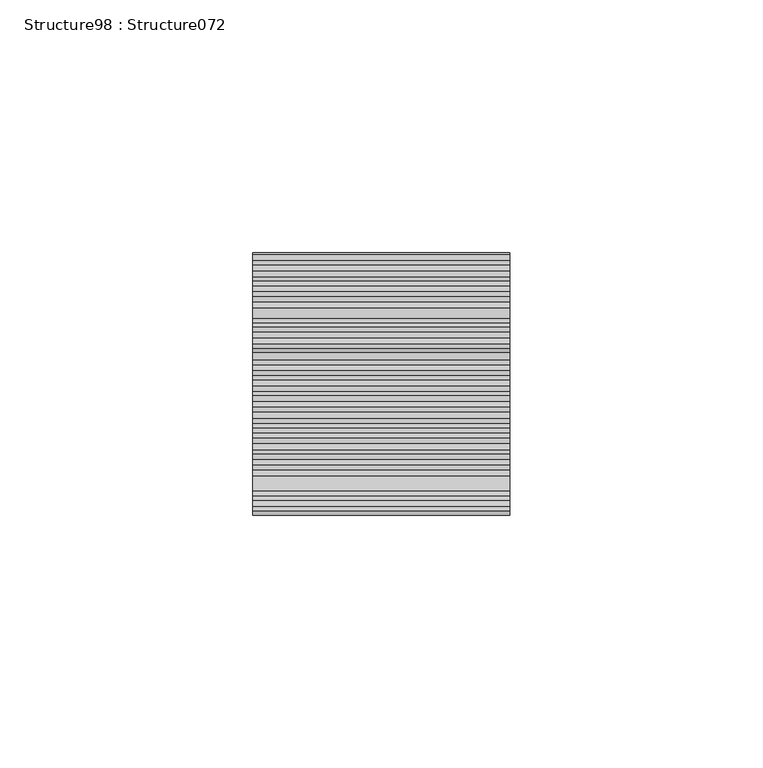
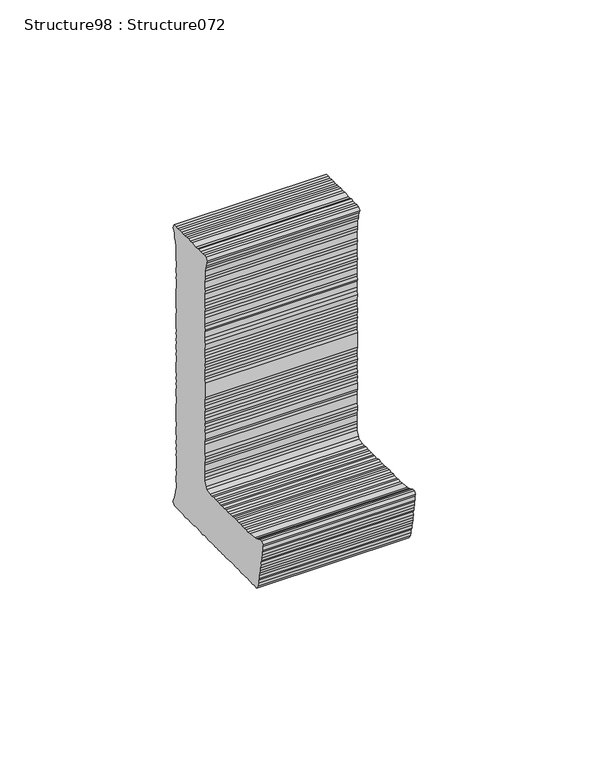
"""IFC4 building model written with IfcOpenShell, lengths in millimetres: proxy geometry, Structure98 : Structure072."""

from ifc_helpers import new_model, si_unit, frame, origin, place, context, project, spatial, polyline, outline, extrude, source, transform, mapped, element, save


def structure98_structure072_e171fc14(model_context):
    return source(origin(), model_context, "Body", "SweptSolid", [
        extrude(outline(polyline([(1.1010062, 0.0), (1.4689097, -0.9240496), (2.4792082, -1.7515268), (2.7518087, -2.5801663), (3.483875, -3.3169318), (4.2109946, -4.4202642), (4.8547815, -5.0681837), (5.0302245, -5.9878436), (5.85945, -6.6330855), (6.4122109, -7.7361117), (7.0502297, -8.378226), (7.6890699, -9.3927123), (8.143826, -10.2224378), (8.8758924, -10.9592033), (9.2425421, -11.8819909), (9.8834908, -12.7092928), (10.6147026, -13.6345048), (10.7949436, -15.0991479), (9.6880807, -15.8287721), (9.2244897, -16.6595852), (8.3060733, -17.3900639), (7.8433384, -18.0319274), (6.921992, -18.5772184), (6.2800313, -19.4031836), (5.3550717, -20.1341446), (4.8038967, -21.0519831), (3.9732372, -21.8773446), (3.234126, -22.2415627), (2.5921653, -23.0675278), (1.8523709, -23.8026037), (1.116714, -24.3454696), (0.377172, -25.0802946), (-0.3597719, -26.1827171), (-1.8320409, -27.6455958), (-2.6622696, -28.1003503), (-3.3080959, -29.1122363), (-4.1386759, -29.7554389), (-4.5981296, -30.394042), (-5.5162936, -31.12427), (-5.9828146, -31.7698953), (-6.901231, -32.500374), (-7.7348205, -33.1405478), (-8.2859955, -34.0583863), (-8.9273526, -34.6956526), (-9.8522326, -35.2444548), (-10.5884933, -35.9760195), (-11.2376008, -36.9911658), (-12.2500648, -37.6269932), (-12.706509, -38.2686252), (-13.6312162, -38.9993355), (-14.4621281, -39.8249478), (-14.8272819, -40.5579514), (-15.6581143, -41.2014047), (-16.4854926, -42.0235059), (-17.2244308, -42.5696321), (-17.6844882, -43.3969341), (-18.4240301, -44.1317591), (-19.5311454, -44.8616342), (-22.4794694, -47.7911534), (-22.9391949, -48.4360456), (-24.1293814, -48.1569864), (-24.7727568, -47.1444983), (-25.1366477, -46.2244871), (-25.6857039, -45.3003612), (-26.3253191, -44.2921623), (-27.2382662, -42.4480253), (-27.8762849, -41.805911), (-28.884634, -41.1555671), (-29.6214084, -40.2388919), (-30.9038644, -38.7588973), (-31.7290772, -38.1176937), (-32.2726955, -37.3812796), (-34.655234, -34.9834473), (-35.2993739, -34.5244791), (-36.1206206, -33.5086544), (-36.9448872, -33.0435746), (-37.5872612, -32.0325993), (-38.5015626, -31.4769067), (-39.6011332, -30.0058001), (-40.6962568, -29.2681246), (-41.2500089, -28.710818), (-42.0740595, -27.7063063), (-42.7114745, -26.8754932), (-44.0879315, -25.6795071), (-45.0951753, -24.8409691), (-45.6486196, -24.1088008), (-46.376981, -23.5509354), (-47.2050443, -22.5423853), (-47.8458217, -21.8974947), (-48.3921987, -21.158304), (-49.2153031, -20.3299161), (-50.2221475, -19.6810866), (-50.7731408, -19.1265564), (-51.4163692, -18.3040276), (-52.2386191, -17.2871932), (-53.0618826, -16.823123), (-53.5204248, -15.9971595), (-54.3499011, -15.3516651), (-55.1681383, -14.3388692), (-56.0809351, -13.784691), (-56.8157601, -13.0451491), (-57.3692044, -12.3129807), (-58.1886039, -11.6634929), (-58.6471462, -10.8375294), (-59.5630441, -9.9157522), (-60.3903203, -9.4476435), (-61.0296846, -8.4396972), (-61.856653, -7.7967268), (-62.5912273, -7.0574373), (-63.0435567, -6.4128979), (-63.873033, -5.7674036), (-64.6942797, -4.7515788), (-65.5145337, -4.2905374), (-66.0668727, -3.370175), (-66.8025522, -2.8190796), (-67.7117358, -2.0792313), (-68.3592276, -1.2524117), (-68.9997543, -0.6077735), (-69.8221633, 0.0447432), (-71.1040607, 1.699347), (-71.9332862, 2.344589), (-72.9325047, 3.1750501), (-73.5732821, 3.8199407), (-74.222028, 4.6480224), (-74.9463767, 5.2018493), (-75.7746907, 6.2106518), (-76.3256841, 6.765182), (-76.9613436, 7.5942283), (-78.6133206, 9.2568094), (-79.3427872, 9.6264807), (-79.9864151, 10.6387179), (-80.7218438, 11.189561), (-81.4564181, 11.9288505), (-82.1836172, 12.850024), (-83.0097311, 13.6814408), (-83.8389566, 14.3266828), (-84.569769, 15.0621863), (-85.2043336, 15.5256528), (-85.9426127, 16.4438424), (-86.8517963, 17.1836906), (-88.4134185, 18.3837916), (-89.4232258, 18.6569901), (-90.4299906, 19.4879785), (-91.3468001, 20.0461951), (-92.1709197, 20.3213156), (-92.8136915, 21.5225025), (-91.9830319, 22.347864), (-91.2516384, 22.8950207), (-90.5105105, 23.8109935), (-89.679851, 24.636355), (-88.9442735, 24.9970619), (-88.3035668, 25.8242891), (-87.6535566, 26.6497254), (-86.9172959, 27.3812901), (-85.9926683, 27.9298414), (-85.3503756, 28.9382164), (-83.6894873, 30.2183324), (-83.0443443, 30.8593606), (-82.6756568, 31.5958754), (-81.7543105, 32.1411664), (-80.9233985, 32.9667787), (-80.2813583, 33.9749028), (-79.4511296, 34.4296573), (-78.3476967, 34.2444712), (-77.893771, 33.2338472), (-77.2536767, 32.2180989), (-76.7984173, 31.3883717), (-76.250423, 30.289638), (-74.8746493, 28.7227941), (-74.2338718, 28.0779034), (-73.50266, 27.1526915), (-71.9459846, 25.5860237), (-71.3015939, 25.126803), (-70.5744743, 24.0234707), (-69.1988718, 22.639038), (-68.3756879, 21.992809), (-67.6409424, 21.0711082), (-66.8141453, 20.6105491), (-66.2696034, 19.6909665), (-65.4432387, 18.8592973), (-64.6203056, 18.2133206), (-63.154919, 16.7385276), (-62.5139703, 15.9112257), (-61.5933764, 15.3562677), (-61.2324153, 14.6214443), (-59.765524, 13.1451369), (-58.9435941, 12.5001698), (-57.9317909, 11.6711782), (-56.6509192, 10.0105392), (-56.0098909, 9.3653961), (-55.1884626, 8.7209339), (-54.4527831, 8.1698384), (-53.6269199, 7.338674), (-52.9905876, 6.3267117), (-52.2513175, 5.9542414), (-51.5241183, 5.0330679), (-50.7923028, 4.2965549), (-50.0575573, 3.374854), (-49.326745, 2.6393506), (-48.408659, 2.0869167), (-44.8386131, -1.5060456), (-44.1984393, -2.3396351), (-43.3739097, -3.3516963), (-42.7358115, -3.8116517), (-41.9063352, -4.4571461), (-41.266241, -5.4728944), (-40.4430571, -6.1191235), (-39.6184479, -6.9490259), (-38.7917304, -7.5917438), (-38.2456042, -8.330682), (-37.5101754, -8.8815251), (-36.6889288, -9.8973498), (-35.8597032, -10.5425918), (-34.3995833, -12.0120844), (-34.0316, -12.753975), (-33.2084161, -13.4002041), (-31.0109632, -15.6117626), (-30.0904489, -16.3488794), (-29.4536841, -16.9897316), (-28.7225518, -18.0971024), (-28.0816948, -18.5598342), (-26.5210067, -20.1305405), (-25.9753595, -20.8619291), (-25.0582076, -21.7849683), (-24.3263126, -22.3393226), (-22.5817702, -22.9869896), (-21.7576522, -23.2626134), (-20.0976184, -22.1709437), (-19.2703197, -21.5310014), (-18.7158633, -20.6099027), (-17.794517, -20.0646117), (-17.1458404, -19.4200723), (-16.4097525, -18.5065995), (-15.5824537, -17.8666572), (-15.1197187, -17.2247938), (-14.1977688, -16.4908039), (-13.555476, -15.482429), (-12.7254998, -15.0279253), (-11.8945082, -14.0201541), (-11.0672095, -13.3802118), (-10.6038708, -12.5496495), (-9.8682138, -12.0067836), (-9.222467, -11.1770565), (-8.3013732, -10.6320163), (-7.5644292, -9.5295939), (-6.9166085, -9.0740041), (-5.9981922, -8.3435253), (-5.3529696, -7.5203382), (-4.5223895, -6.8771355), (-3.7825156, -5.9599008), (-1.943986, -3.5753213), (-1.4766346, -2.7487976), (-1.0201108, -1.9250067), (-0.550319, -0.7288888), (0.0, 0.0), (1.1010062, 0.0)])), frame((-56111.5043079, 291302.7385981, -357.2810245), z_axis=(-0.9999998917542983, 0.0004652863545059615, 0.0), x_axis=(-0.0003300580295796821, -0.7093652987222075, -0.7048409494562944)), (0.0, 0.0, 1.0), 50.8),
    ])


if __name__ == "__main__":
    model = new_model("IFC4")
    model_context = context("Model", 3, world=origin())
    ifc_project = project(units=[si_unit("LENGTHUNIT", "METRE", prefix="MILLI")], contexts=[model_context])
    site = spatial("IfcSite", under=ifc_project)
    building = spatial("IfcBuilding", under=site)
    placement = place(None, origin())
    structure98_structure072_shape = structure98_structure072_e171fc14(model_context)
    element("IfcBuildingElementProxy", 1, Name="Structure98 : Structure072", ObjectType="Structure98 : Structure072", at=placement, inside=building, context=model_context, shape_type="MappedRepresentation", body=[
        mapped(structure98_structure072_shape, transform((0.0, 0.0, 0.0), x_axis=(1.0, 0.0, 0.0), y_axis=(0.0, 1.0, 0.0), z_axis=(0.0, 0.0, 1.0))),
    ])
    save(model, "model.ifc")

# Revit data of these elements
# Type "Structure98 : Structure072"
#   NameOverride = "Structure072"
# Element 1 (IfcBuildingElementProxy, "Structure98 : Structure072")
#   Materials on its faces: "BRUSHED ALUMINUM LETTERING"
# Materials
#   "BRUSHED ALUMINUM LETTERING": class "Unassigned", colour RGB 169 181 186, transparency 0, Cost = 0
